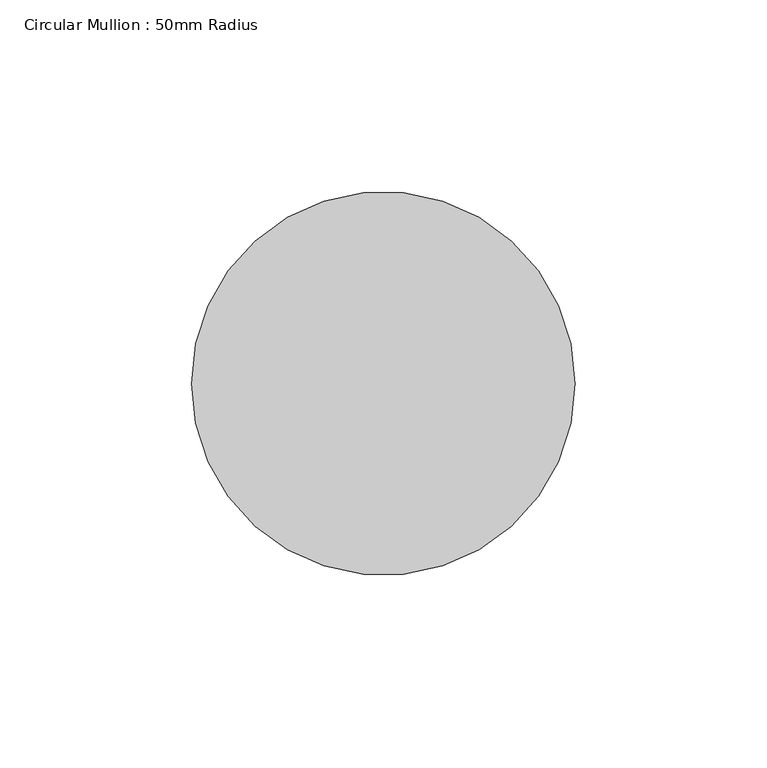
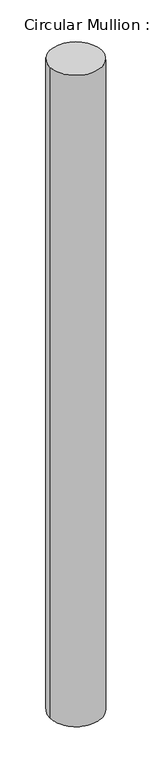
"""IFC4 building model written with IfcOpenShell, lengths in millimetres: member geometry, Circular Mullion : 50mm Radius."""

from ifc_helpers import new_model, si_unit, frame, origin, place, context, project, spatial, ellipse_curve, source, transform, mapped, element, save
from ifc_brep_helpers import plane_surface, cylinder_surface, advanced_brep


def circular_mullion_50mm_radius_dfca9b12(model_context):
    return source(origin(), model_context, "Body", "AdvancedBrep", [
        advanced_brep(
        [(-100.0, 0.0, 0.5449018), (0.0, 0.0, 0.0), (0.0, 0.0, -1327.2663867), (-100.0, 0.0, -1327.8472335)],
        [
            (0, 1, ellipse_curve(frame((-50.0, 0.0, 0.2724509), z_axis=(-0.0054482648441654775, -0.015709827997784618, -0.9998617493006061), x_axis=(-0.32761555201683906, -0.9446647912308207, 0.016627756479202168)), 50.0069135, 50.0)),
            (1, 2),
            (2, 3, ellipse_curve(frame((-50.0, 0.0, -1327.5568101), z_axis=(-0.005807555678420319, -0.01674582704863214, 0.9998429124485002), x_axis=(0.32760937991784983, 0.9446469942594118, 0.01772428916771619)), 50.0078556, 50.0)),
            (3, 0),
            (1, 0, ellipse_curve(frame((-50.0, 0.0, 0.2724509), z_axis=(-0.0054482648441654775, -0.015709827997784618, -0.9998617493006061), x_axis=(-0.32761555201683906, -0.9446647912308207, 0.016627756479202168)), 50.0069135, 50.0)),
            (3, 2, ellipse_curve(frame((-50.0, 0.0, -1327.5568101), z_axis=(-0.005807555678420319, -0.01674582704863214, 0.9998429124485002), x_axis=(0.32760937991784983, 0.9446469942594118, 0.01772428916771619)), 50.0078556, 50.0)),
        ],
        [
            cylinder_surface(frame((-50.0, 0.0, 0.0), z_axis=(0.0, 0.0, 1.0), x_axis=(1.0, 0.0, 0.0)), 50.0),
            plane_surface(frame((-287.9736409, 99.8710275, 0.0), z_axis=(0.0054482648441654775, 0.015709827997784618, 0.9998617493006061), x_axis=(0.3276155520168401, 0.9446647912308203, -0.016627756479217118))),
            plane_surface(frame((-287.9736409, 99.8710275, -1327.2663867), z_axis=(0.00580755567842032, 0.016745827048632145, -0.9998429124485004), x_axis=(0.32760937991784994, 0.9446469942594119, 0.017724289167711408))),
        ],
        [
            (0, [[1, 2, 3, 4]]),
            (0, [[5, -4, 6, -2]]),
            (1, [[-1, -5]]),
            (2, [[-6, -3]]),
        ],
    ),
    ])


if __name__ == "__main__":
    model = new_model("IFC4")
    model_context = context("Model", 3, world=origin())
    ifc_project = project(units=[si_unit("LENGTHUNIT", "METRE", prefix="MILLI")], contexts=[model_context])
    site = spatial("IfcSite", under=ifc_project)
    building = spatial("IfcBuilding", under=site)
    placement = place(None, origin())
    circular_mullion_50mm_radius_shape = circular_mullion_50mm_radius_dfca9b12(model_context)
    element("IfcMember", 1, ObjectType="Circular Mullion : 50mm Radius", at=placement, inside=building, context=model_context, shape_type="MappedRepresentation", body=[
        mapped(circular_mullion_50mm_radius_shape, transform((0.0, 0.0, 0.0), x_axis=(1.0, 0.0, 0.0), y_axis=(0.0, 1.0, 0.0), z_axis=(0.0, 0.0, 1.0))),
    ])
    save(model, "model.ifc")

# Revit data of these elements
# Type "Circular Mullion : 50mm Radius"
#   built-in parameter 1007350 = 0.164042 (stored number, unit not read)
# Element 1 (IfcMember, "Circular Mullion : 50mm Radius")
#   Materials on its faces: "Aluminium"
# Materials
#   "Aluminium": class "Metal", colour RGB 247 247 247, transparency 0, Description = "Aluminium 6061", Cost = 0
